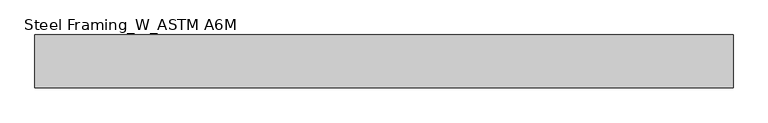
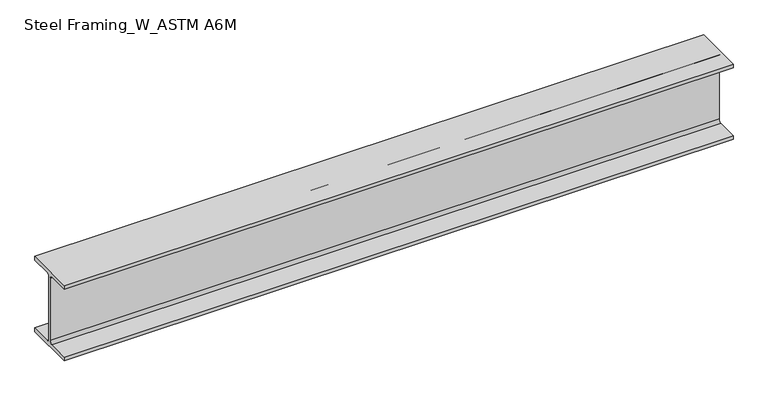
"""IFC4 building model written with IfcOpenShell, lengths in millimetres: beam geometry, Steel Framing_W_ASTM A6M : H_SB_AR_S02_W200x31.3_B6."""

from ifc_helpers import new_model, si_unit, point, frame, frame_2d, origin, place, context, project, spatial, polyline, circle_curve, trimmed, segment, composite_curve, outline, extrude, source, transform, mapped, element, save


def steel_framing_w_astm_a6m_cb9fb0c6(model_context):
    return source(origin(), model_context, "Body", "SweptSolid", [
        extrude(outline(composite_curve([segment(polyline([(67.0, -94.8), (67.0, -105.0), (-67.0, -105.0), (-67.0, -94.8), (-10.775, -94.8)]), True, "CONTINUOUS"), segment(trimmed(circle_curve(frame_2d((-10.775, -87.2)), 7.6), [point((-10.775, -94.8))], [point((-3.175, -87.2))], True, "CARTESIAN"), True, "CONTINUOUS"), segment(polyline([(-3.175, -87.2), (-3.175, 87.2)]), True, "CONTINUOUS"), segment(trimmed(circle_curve(frame_2d((-10.775, 87.2)), 7.6), [point((-3.175, 87.2))], [point((-10.775, 94.8))], True, "CARTESIAN"), True, "CONTINUOUS"), segment(polyline([(-10.775, 94.8), (-67.0, 94.8), (-67.0, 105.0), (67.0, 105.0), (67.0, 94.8), (10.775, 94.8)]), True, "CONTINUOUS"), segment(trimmed(circle_curve(frame_2d((10.775, 87.2)), 7.6), [point((10.775, 94.8))], [point((3.175, 87.2))], True, "CARTESIAN"), True, "CONTINUOUS"), segment(polyline([(3.175, 87.2), (3.175, -87.2)]), True, "CONTINUOUS"), segment(trimmed(circle_curve(frame_2d((10.775, -87.2)), 7.6), [point((3.175, -87.2))], [point((10.775, -94.8))], True, "CARTESIAN"), True, "CONTINUOUS"), segment(polyline([(10.775, -94.8), (67.0, -94.8)]), True, "CONTINUOUS")], self_intersect=False)), frame((-846.3, 0.0, 0.0), z_axis=(1.0, 0.0, 0.0), x_axis=(0.0, 1.0, 0.0)), (0.0, 0.0, 1.0), 1766.6),
    ])


if __name__ == "__main__":
    model = new_model("IFC4")
    model_context = context("Model", 3, world=origin())
    ifc_project = project(units=[si_unit("LENGTHUNIT", "METRE", prefix="MILLI")], contexts=[model_context])
    site = spatial("IfcSite", under=ifc_project)
    building = spatial("IfcBuilding", under=site)
    placement = place(None, origin())
    steel_framing_w_astm_a6m_shape = steel_framing_w_astm_a6m_cb9fb0c6(model_context)
    element("IfcBeam", 1, ObjectType="Steel Framing_W_ASTM A6M : H_SB_AR_S02_W200x31.3_B6", at=placement, inside=building, context=model_context, shape_type="MappedRepresentation", body=[
        mapped(steel_framing_w_astm_a6m_shape, transform((0.0, 0.0, 0.0), x_axis=(1.0, 0.0, 0.0), y_axis=(0.0, 1.0, 0.0), z_axis=(0.0, 0.0, 1.0))),
    ])
    save(model, "model.ifc")

# Revit data of these elements
# Type "Steel Framing_W_ASTM A6M : H_SB_AR_S02_W200x31.3_B6"
#   Type Mark = "B6"
#   Section Name Key = "W8x21"
#   Width = 13.4 cm
#   Web Thickness = 0.635 cm
#   Web Fillet = 0.76 cm
#   Warping Constant = 40800.0 cm⁶
#   Torsional Moment of Inertia = 11.70 cm⁴
#   Section Area = 39.7 cm²
#   Plastic Modulus weak axis = 93.2 cm³
#   Plastic Modulus strong axis = 334.0 cm³
#   Perimeter = 0.93 m²/m
#   Nominal Weight = 31.30 kgf/m
#   Moment of Inertia weak axis = 407.00 cm⁴
#   Moment of Inertia strong axis = 3130.00 cm⁴
#   Height = 21.0 cm
#   Flange Thickness = 1.02 cm
#   Elastic Modulus weak axis = 60.8 cm³
#   Elastic Modulus strong axis = 298.0 cm³
#   Centroid Vertical = 10.5 cm
#   Centroid Horizontal = 6.7 cm
#   Length [instance default] = 1500 mm
#   Structural Material [instance default] = Steel, 45-345
#   Bolt Spacing = 0
#   Assembly Code = ""
# Element 1 (IfcBeam, "Steel Framing_W_ASTM A6M : H_SB_AR_S02_W200x31.3_B6")
#   Materials on its faces: "Steel, 45-345"
# Materials
#   "Steel, 45-345": class "Metal", colour RGB 189 187 185, transparency 0, Description = "Steel 345 MPa", Cost = 0
